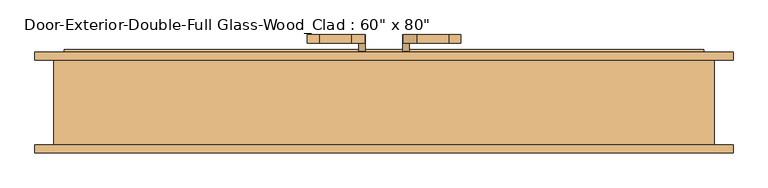
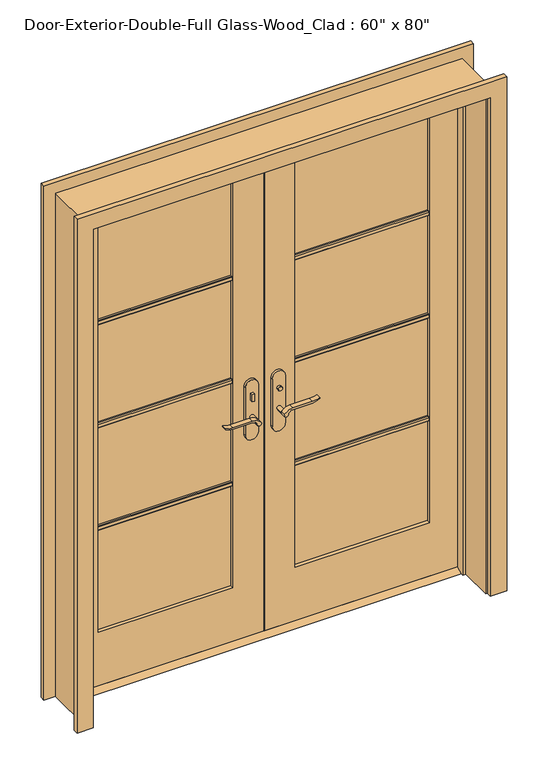
"""IFC4 building model written with IfcOpenShell, lengths in millimetres: door geometry."""

import ifcopenshell
import ifcopenshell.guid

model = None  # the IFC model being written
_history = None  # IfcOwnerHistory: only IFC2X3 demands one
_inside = {}  # id of a spatial element -> (the spatial element, [elements in it])
_under = {}  # id of a project, library or spatial element -> (it, [spatial elements below it])
_declared = {}  # id of a project -> (the project, [libraries it declares])
_typed = {}  # id of a type object -> (the type object, [elements of that type])
_made_of = {}  # id of a material, layer set ... -> (it, [elements and type objects made of it])


def new_model(schema):
    """Start an empty IFC model of exactly this schema.

    Asked for "IFC4X3", IfcOpenShell would pick the latest addendum, in which some entities
    have other attributes; the version numbers below select the first issue.
    IFC2X3 requires an IfcOwnerHistory on every rooted entity: one is made here for all.
    """
    global model, _history
    if schema == "IFC4X3":
        model = ifcopenshell.file(schema_version=(4, 3, 0, 0))
    else:
        model = ifcopenshell.file(schema=schema)
    _inside.clear()
    _under.clear()
    _declared.clear()
    _typed.clear()
    _made_of.clear()
    _history = None
    if model.schema == "IFC2X3":
        org = make("IfcOrganization", Name="unknown")
        user = make(
            "IfcPersonAndOrganization",
            ThePerson=make("IfcPerson", FamilyName="unknown"),
            TheOrganization=org,
        )
        app = make(
            "IfcApplication",
            ApplicationDeveloper=org,
            Version="unknown",
            ApplicationFullName="unknown",
            ApplicationIdentifier="unknown",
        )
        _history = make(
            "IfcOwnerHistory",
            OwningUser=user,
            OwningApplication=app,
            ChangeAction="ADDED",
            CreationDate=0,
        )
    return model


def make(cls, **values):
    """One entity of the class cls with the attributes given. An attribute that is None is left unset."""
    return model.create_entity(
        cls, **{name: value for name, value in values.items() if value is not None}
    )


def rooted(cls, **values):
    """An entity with a GlobalId (a new one), such as an element, a storey or a relation."""
    return make(cls, GlobalId=ifcopenshell.guid.new(), OwnerHistory=_history, **values)


def si_unit(unit_type, name, prefix=None):
    """IfcSIUnit, for example si_unit("LENGTHUNIT", "METRE", prefix="MILLI")."""
    return make("IfcSIUnit", UnitType=unit_type, Prefix=prefix, Name=name)


def assignment(units):
    """IfcUnitAssignment: the units of a project."""
    return None if units is None else make("IfcUnitAssignment", Units=units)


def point(xyz):
    """IfcCartesianPoint."""
    return None if xyz is None else make("IfcCartesianPoint", Coordinates=xyz)


def direction(xyz):
    """IfcDirection."""
    return None if xyz is None else make("IfcDirection", DirectionRatios=xyz)


def frame(location, z_axis=None, x_axis=None):
    """IfcAxis2Placement3D, a coordinate frame: its origin and axes. An axis left out is left unset."""
    return make(
        "IfcAxis2Placement3D",
        Location=point(location),
        Axis=direction(z_axis),
        RefDirection=direction(x_axis),
    )


def frame_2d(location, x_axis=None):
    """IfcAxis2Placement2D, a coordinate frame in the plane: its origin and x axis."""
    return make(
        "IfcAxis2Placement2D", Location=point(location), RefDirection=direction(x_axis)
    )


def origin():
    """The frame at (0, 0, 0) with its axes left unset."""
    return frame((0.0, 0.0, 0.0))


def place(relative_to, where):
    """IfcLocalPlacement: puts the frame where relative to a parent placement (None: the world)."""
    return make(
        "IfcLocalPlacement", PlacementRelTo=relative_to, RelativePlacement=where
    )


def context(
    kind, dimensions, precision=None, world=None, true_north=None, identifier=None
):
    """IfcGeometricRepresentationContext, for example the 3D "Model" context."""
    return make(
        "IfcGeometricRepresentationContext",
        ContextIdentifier=identifier,
        ContextType=kind,
        CoordinateSpaceDimension=dimensions,
        Precision=precision,
        WorldCoordinateSystem=world,
        TrueNorth=true_north,
    )


def project(units=None, contexts=None):
    """IfcProject with its units and contexts."""
    return rooted(
        "IfcProject",
        Name="project",
        RepresentationContexts=contexts,
        UnitsInContext=assignment(units),
    )


def spatial(cls, under=None, at=None, **own):
    """A site, building, storey or space (cls), placed at a placement, below another one or the project."""
    s = rooted(cls, ObjectPlacement=at, **own)
    if under is not None:
        _under.setdefault(under.id(), (under, []))[1].append(s)
    return s


def polyline(points):
    """IfcPolyline through the points."""
    return make("IfcPolyline", Points=[point(p) for p in points])


def circle_curve(where, radius):
    """IfcCircle in the frame where."""
    return make("IfcCircle", Position=where, Radius=radius)


def trimmed(basis, trim1, trim2, sense, master):
    """IfcTrimmedCurve: the piece of a basis curve between two trims."""
    return make(
        "IfcTrimmedCurve",
        BasisCurve=basis,
        Trim1=trim1,
        Trim2=trim2,
        SenseAgreement=sense,
        MasterRepresentation=master,
    )


def segment(curve, same_sense, transition):
    """IfcCompositeCurveSegment."""
    return make(
        "IfcCompositeCurveSegment",
        Transition=transition,
        SameSense=same_sense,
        ParentCurve=curve,
    )


def composite_curve(segments, self_intersect=None):
    """IfcCompositeCurve: segments joined end to end."""
    return make("IfcCompositeCurve", Segments=segments, SelfIntersect=self_intersect)


def outline(outer, holes=None, kind="AREA"):
    """IfcArbitraryClosedProfileDef: a profile drawn as a closed curve; with holes, ...WithVoids."""
    if holes is None:
        return make("IfcArbitraryClosedProfileDef", ProfileType=kind, OuterCurve=outer)
    return make(
        "IfcArbitraryProfileDefWithVoids",
        ProfileType=kind,
        OuterCurve=outer,
        InnerCurves=holes,
    )


def extrude(swept, where, along, depth):
    """IfcExtrudedAreaSolid: the profile swept, set in the frame where, extruded along a direction by depth."""
    return make(
        "IfcExtrudedAreaSolid",
        SweptArea=swept,
        Position=where,
        ExtrudedDirection=direction(along),
        Depth=depth,
    )


def faces_of(points, faces, orient=None, outer=None):
    """IfcFace entities. A face is a list of loops; a loop is a list of indices into points, from 0.

    orient and outer hold one flag for each loop. By default every Orientation is true, the
    first loop of a face is its IfcFaceOuterBound and the others are IfcFaceBound.
    """
    made = []
    for i, loops in enumerate(faces):
        bounds = []
        for j, loop in enumerate(loops):
            is_outer = j == 0 if outer is None else outer[i][j]
            bounds.append(
                make(
                    "IfcFaceOuterBound" if is_outer else "IfcFaceBound",
                    Bound=make("IfcPolyLoop", Polygon=[points[k] for k in loop]),
                    Orientation=True if orient is None else orient[i][j],
                )
            )
        made.append(make("IfcFace", Bounds=bounds))
    return made


def faceted_brep(points, faces, orient=None, outer=None, voids=None):
    """IfcFacetedBrep: a solid bounded by flat faces; with voids (closed shells), ...WithVoids."""
    shared = [point(p) for p in points]
    hull = make("IfcClosedShell", CfsFaces=faces_of(shared, faces, orient, outer))
    if voids is None:
        return make("IfcFacetedBrep", Outer=hull)
    return make(
        "IfcFacetedBrepWithVoids",
        Outer=hull,
        Voids=[
            make(cls, CfsFaces=faces_of(shared, fs, o, b)) for cls, fs, o, b in voids
        ],
    )


def shape(context_of_items, identifier, shape_type, items):
    """IfcShapeRepresentation: the items that make up one representation, for example the "Body"."""
    return make(
        "IfcShapeRepresentation",
        ContextOfItems=context_of_items,
        RepresentationIdentifier=identifier,
        RepresentationType=shape_type,
        Items=items,
    )


def source(mapping_origin, context_of_items, identifier, shape_type, items):
    """IfcRepresentationMap: a shape defined once, which mapped items show again and again."""
    return make(
        "IfcRepresentationMap",
        MappingOrigin=mapping_origin,
        MappedRepresentation=shape(context_of_items, identifier, shape_type, items),
    )


def transform(
    local_origin,
    x_axis=None,
    y_axis=None,
    z_axis=None,
    scale=None,
    scale2=None,
    scale3=None,
    uniform=True,
):
    """IfcCartesianTransformationOperator3D, or its non-uniform kind. x_axis, y_axis, z_axis: its Axis1, 2, 3."""
    if uniform:
        return make(
            "IfcCartesianTransformationOperator3D",
            Axis1=direction(x_axis),
            Axis2=direction(y_axis),
            LocalOrigin=point(local_origin),
            Scale=scale,
            Axis3=direction(z_axis),
        )
    return make(
        "IfcCartesianTransformationOperator3DnonUniform",
        Axis1=direction(x_axis),
        Axis2=direction(y_axis),
        LocalOrigin=point(local_origin),
        Scale=scale,
        Axis3=direction(z_axis),
        Scale2=scale2,
        Scale3=scale3,
    )


def mapped(mapping_source, mapping_target):
    """IfcMappedItem: shows the shape of a source again, moved by a transform."""
    return make(
        "IfcMappedItem", MappingSource=mapping_source, MappingTarget=mapping_target
    )


def made_of(thing, what):
    """Note that an element or type object is made of a material, layer set ...; save() writes the relation."""
    if what is not None:
        _made_of.setdefault(what.id(), (what, []))[1].append(thing)
    return thing


def element(
    cls,
    number,
    at=None,
    inside=None,
    cuts=None,
    type_object=None,
    material=None,
    context=None,
    identifier="Body",
    shape_type=None,
    held_by="IfcProductDefinitionShape",
    body=None,
    shapes=None,
    **own,
):
    """One element of the class cls, such as IfcWall. Its Tag is "e" and its number.

    at: its placement. inside: the storey or other place that contains it. cuts: it is an
    opening in that element (IfcRelVoidsElement). A single representation is given by context,
    identifier, shape_type and body (its items); several are given by shapes. held_by: the class
    of the entity that holds the representations. save() writes the other relations.
    """
    e = rooted(cls, Tag="e%d" % number, ObjectPlacement=at, **own)
    if body is not None:
        shapes = [shape(context, identifier, shape_type, body)]
    if shapes is not None:
        e.Representation = make(held_by, Representations=shapes)
    if inside is not None:
        _inside.setdefault(inside.id(), (inside, []))[1].append(e)
    if cuts is not None:
        rooted(
            "IfcRelVoidsElement", RelatingBuildingElement=cuts, RelatedOpeningElement=e
        )
    if type_object is not None:
        _typed.setdefault(type_object.id(), (type_object, []))[1].append(e)
    return made_of(e, material)


def aggregate(whole, parts):
    """IfcRelAggregates: a whole, such as a stair, and the parts it consists of."""
    return rooted("IfcRelAggregates", RelatingObject=whole, RelatedObjects=parts)


def save(model, path):
    """Write the relations noted so far, then the file.

    IfcRelAggregates (storeys below a building ...), IfcRelContainedInSpatialStructure (elements
    in a storey), IfcRelDefinesByType, IfcRelAssociatesMaterial and IfcRelDeclares: one each for
    every whole, place, type object, material and project.
    """
    for whole, parts in _under.values():
        aggregate(whole, parts)
    for where, things in _inside.values():
        rooted(
            "IfcRelContainedInSpatialStructure",
            RelatedElements=things,
            RelatingStructure=where,
        )
    for kind, things in _typed.values():
        rooted("IfcRelDefinesByType", RelatedObjects=things, RelatingType=kind)
    for what, things in _made_of.values():
        rooted("IfcRelAssociatesMaterial", RelatedObjects=things, RelatingMaterial=what)
    for by, libraries in _declared.values():
        rooted("IfcRelDeclares", RelatingContext=by, RelatedDefinitions=libraries)
    model.write(path)


def door_b03bd389(model_context):
    return source(origin(), model_context, "Body", "SolidModel", [
        extrude(outline(polyline([(63.5, 12.7), (98.425, 12.7), (123.825, 0.0), (38.1, 0.0), (63.5, 12.7)])), frame((-762.0, 0.0, 0.0), z_axis=(1.0, 0.0, 0.0), x_axis=(0.0, 1.0, 0.0)), (0.0, 0.0, 1.0), 1524.0),
        extrude(outline(polyline([(-47.4019111, 43.5), (-57.4019111, 43.5), (-57.4019111, 53.5), (-47.4019111, 53.5), (-47.4019111, 43.5)])), frame((0.0, 0.0, 981.9), z_axis=(0.0, 0.0, 1.0), x_axis=(1.0, 0.0, 0.0)), (0.0, 0.0, 1.0), 30.0),
        extrude(outline(composite_curve([segment(trimmed(circle_curve(frame_2d((996.9, -52.4019111)), 8.0), [point((996.9, -60.4019111))], [point((996.9, -44.4019111))], False, "CARTESIAN"), True, "CONTINUOUS"), segment(trimmed(circle_curve(frame_2d((996.9, -52.4019111)), 8.0), [point((996.9, -44.4019111))], [point((996.9, -60.4019111))], False, "CARTESIAN"), True, "CONTINUOUS")], self_intersect=False)), frame((0.0, 108.425, 0.0), z_axis=(0.0, 1.0, 0.0), x_axis=(0.0, 0.0, 1.0)), (0.0, 0.0, 1.0), 10.0),
        extrude(outline(composite_curve([segment(trimmed(circle_curve(frame_2d((897.1555521, -76.0694241)), 37.2832219), [point((919.0523287, -45.8937749))], [point((934.4, -77.7693445))], False, "CARTESIAN"), True, "CONTINUOUS"), segment(polyline([(934.4, -77.7693445), (934.4, -154.045502)]), True, "CONTINUOUS"), segment(trimmed(circle_curve(frame_2d((1017.6850638, -153.9791202)), 83.2850902), [point((934.4, -154.045502))], [point((939.4, -182.4019111))], True, "CARTESIAN"), True, "CONTINUOUS"), segment(polyline([(939.4, -182.4019111), (936.6135558, -182.4019111)]), True, "CONTINUOUS"), segment(trimmed(circle_curve(frame_2d((986.6709207, -150.4622499)), 59.3791355), [point((936.6135558, -182.4019111))], [point((927.4, -154.045502))], False, "CARTESIAN"), True, "CONTINUOUS"), segment(polyline([(927.4, -154.045502), (927.4, -77.7881013)]), True, "CONTINUOUS"), segment(trimmed(circle_curve(frame_2d((909.2738613, -77.7881013)), 18.1261387), [point((927.4, -77.7881013))], [point((914.4, -60.4019111))], True, "CARTESIAN"), True, "CONTINUOUS"), segment(trimmed(circle_curve(frame_2d((914.4, -52.4019111)), 8.0), [point((914.4, -60.4019111))], [point((919.0523287, -45.8937749))], False, "CARTESIAN"), True, "CONTINUOUS")], self_intersect=False)), frame((0.0, 3.5, 0.0), z_axis=(0.0, 1.0, 0.0), x_axis=(0.0, 0.0, 1.0)), (0.0, 0.0, 1.0), 20.0),
        extrude(outline(composite_curve([segment(trimmed(circle_curve(frame_2d((914.4, -52.4019111)), 8.0), [point((914.3999903, -60.4019111))], [point((919.0523287, -45.8937749))], False, "CARTESIAN"), True, "CONTINUOUS"), segment(trimmed(circle_curve(frame_2d((897.1555521, -76.0694241)), 37.2832219), [point((919.0523287, -45.8937749))], [point((934.4, -77.7693445))], False, "CARTESIAN"), True, "CONTINUOUS"), segment(polyline([(934.4, -77.7693445), (934.4, -154.045502)]), True, "CONTINUOUS"), segment(trimmed(circle_curve(frame_2d((1017.6850638, -153.9791202)), 83.2850902), [point((934.4, -154.045502))], [point((939.4, -182.4019111))], True, "CARTESIAN"), True, "CONTINUOUS"), segment(polyline([(939.4, -182.4019111), (936.6135558, -182.4019111)]), True, "CONTINUOUS"), segment(trimmed(circle_curve(frame_2d((986.6709207, -150.4622499)), 59.3791355), [point((936.6135558, -182.4019111))], [point((927.4, -154.045502))], False, "CARTESIAN"), True, "CONTINUOUS"), segment(polyline([(927.4, -154.045502), (927.4, -77.788099)]), True, "CONTINUOUS"), segment(trimmed(circle_curve(frame_2d((909.2738682, -77.788099)), 18.1261318), [point((927.4, -77.788099))], [point((914.3999903, -60.4019111))], True, "CARTESIAN"), True, "CONTINUOUS")], self_intersect=False)), frame((0.0, 138.425, 0.0), z_axis=(0.0, 1.0, 0.0), x_axis=(0.0, 0.0, 1.0)), (0.0, 0.0, 1.0), 20.0),
        extrude(outline(composite_curve([segment(trimmed(circle_curve(frame_2d((914.4, -52.4019111)), 8.0), [point((914.4, -60.4019111))], [point((914.4, -44.4019111))], False, "CARTESIAN"), True, "CONTINUOUS"), segment(trimmed(circle_curve(frame_2d((914.4, -52.4019111)), 8.0), [point((914.4, -44.4019111))], [point((914.4, -60.4019111))], False, "CARTESIAN"), True, "CONTINUOUS")], self_intersect=False)), frame((0.0, 23.5, 0.0), z_axis=(0.0, 1.0, 0.0), x_axis=(0.0, 0.0, 1.0)), (0.0, 0.0, 1.0), 30.0),
        extrude(outline(composite_curve([segment(trimmed(circle_curve(frame_2d((914.4, -52.4019111)), 8.0), [point((914.4, -60.4019111))], [point((914.4, -44.4019111))], False, "CARTESIAN"), True, "CONTINUOUS"), segment(trimmed(circle_curve(frame_2d((914.4, -52.4019111)), 8.0), [point((914.4, -44.4019111))], [point((914.4, -60.4019111))], False, "CARTESIAN"), True, "CONTINUOUS")], self_intersect=False)), frame((0.0, 108.425, 0.0), z_axis=(0.0, 1.0, 0.0), x_axis=(0.0, 0.0, 1.0)), (0.0, 0.0, 1.0), 30.0),
        extrude(outline(composite_curve([segment(polyline([(844.4, -27.4019111), (1039.4, -27.4019111)]), True, "CONTINUOUS"), segment(trimmed(circle_curve(frame_2d((1039.4, -52.4019111)), 25.0), [point((1039.4, -27.4019111))], [point((1039.4, -77.4019111))], False, "CARTESIAN"), True, "CONTINUOUS"), segment(polyline([(1039.4, -77.4019111), (844.4, -77.4019111)]), True, "CONTINUOUS"), segment(trimmed(circle_curve(frame_2d((844.4, -52.4019111)), 25.0), [point((844.4, -77.4019111))], [point((844.4, -27.4019111))], False, "CARTESIAN"), True, "CONTINUOUS")], self_intersect=False)), frame((0.0, 53.5, 0.0), z_axis=(0.0, 1.0, 0.0), x_axis=(0.0, 0.0, 1.0)), (0.0, 0.0, 1.0), 10.0),
        extrude(outline(composite_curve([segment(polyline([(844.4, -27.4019111), (1039.4, -27.4019111)]), True, "CONTINUOUS"), segment(trimmed(circle_curve(frame_2d((1039.4, -52.4019111)), 25.0), [point((1039.4, -27.4019111))], [point((1039.4, -77.4019111))], False, "CARTESIAN"), True, "CONTINUOUS"), segment(polyline([(1039.4, -77.4019111), (844.4, -77.4019111)]), True, "CONTINUOUS"), segment(trimmed(circle_curve(frame_2d((844.4, -52.4019111)), 25.0), [point((844.4, -77.4019111))], [point((844.4, -27.4019111))], False, "CARTESIAN"), True, "CONTINUOUS")], self_intersect=False)), frame((0.0, 98.425, 0.0), z_axis=(0.0, 1.0, 0.0), x_axis=(0.0, 0.0, 1.0)), (0.0, 0.0, 1.0), 10.0),
        extrude(outline(polyline([(47.3875, 118.425), (57.3875, 118.425), (57.3875, 108.425), (47.3875, 108.425), (47.3875, 118.425)])), frame((0.0, 0.0, 981.9), z_axis=(0.0, 0.0, 1.0), x_axis=(1.0, 0.0, 0.0)), (0.0, 0.0, 1.0), 30.0),
        extrude(outline(composite_curve([segment(trimmed(circle_curve(frame_2d((996.9, 52.3875)), 8.0), [point((996.9, 60.3875))], [point((996.9, 44.3875))], False, "CARTESIAN"), True, "CONTINUOUS"), segment(trimmed(circle_curve(frame_2d((996.9, 52.3875)), 8.0), [point((996.9, 44.3875))], [point((996.9, 60.3875))], False, "CARTESIAN"), True, "CONTINUOUS")], self_intersect=False)), frame((0.0, 43.5, 0.0), z_axis=(0.0, 1.0, 0.0), x_axis=(0.0, 0.0, 1.0)), (0.0, 0.0, 1.0), 10.0),
        extrude(outline(composite_curve([segment(trimmed(circle_curve(frame_2d((914.4, 52.3875)), 8.0), [point((919.0523287, 45.8793637))], [point((914.4, 60.3875))], False, "CARTESIAN"), True, "CONTINUOUS"), segment(trimmed(circle_curve(frame_2d((909.2738613, 77.7736901)), 18.1261387), [point((914.4, 60.3875))], [point((927.4, 77.7736901))], True, "CARTESIAN"), True, "CONTINUOUS"), segment(polyline([(927.4, 77.7736901), (927.4, 154.0310909)]), True, "CONTINUOUS"), segment(trimmed(circle_curve(frame_2d((986.6709207, 150.4478388)), 59.3791355), [point((927.4, 154.0310909))], [point((936.6135558, 182.3875))], False, "CARTESIAN"), True, "CONTINUOUS"), segment(polyline([(936.6135558, 182.3875), (939.4, 182.3875)]), True, "CONTINUOUS"), segment(trimmed(circle_curve(frame_2d((1017.6850638, 153.9647091)), 83.2850902), [point((939.4, 182.3875))], [point((934.4, 154.0310909))], True, "CARTESIAN"), True, "CONTINUOUS"), segment(polyline([(934.4, 154.0310909), (934.4, 77.7549333)]), True, "CONTINUOUS"), segment(trimmed(circle_curve(frame_2d((897.1555521, 76.0550129)), 37.2832219), [point((934.4, 77.7549333))], [point((919.0523287, 45.8793637))], False, "CARTESIAN"), True, "CONTINUOUS")], self_intersect=False)), frame((0.0, 138.425, 0.0), z_axis=(0.0, 1.0, 0.0), x_axis=(0.0, 0.0, 1.0)), (0.0, 0.0, 1.0), 20.0),
        extrude(outline(composite_curve([segment(trimmed(circle_curve(frame_2d((909.2738682, 77.7736878)), 18.1261318), [point((914.3999903, 60.3875))], [point((927.4, 77.7736878))], True, "CARTESIAN"), True, "CONTINUOUS"), segment(polyline([(927.4, 77.7736878), (927.4, 154.0310909)]), True, "CONTINUOUS"), segment(trimmed(circle_curve(frame_2d((986.6709207, 150.4478388)), 59.3791355), [point((927.4, 154.0310909))], [point((936.6135558, 182.3875))], False, "CARTESIAN"), True, "CONTINUOUS"), segment(polyline([(936.6135558, 182.3875), (939.4, 182.3875)]), True, "CONTINUOUS"), segment(trimmed(circle_curve(frame_2d((1017.6850638, 153.9647091)), 83.2850902), [point((939.4, 182.3875))], [point((934.4, 154.0310909))], True, "CARTESIAN"), True, "CONTINUOUS"), segment(polyline([(934.4, 154.0310909), (934.4, 77.7549333)]), True, "CONTINUOUS"), segment(trimmed(circle_curve(frame_2d((897.1555521, 76.0550129)), 37.2832219), [point((934.4, 77.7549333))], [point((919.0523287, 45.8793637))], False, "CARTESIAN"), True, "CONTINUOUS"), segment(trimmed(circle_curve(frame_2d((914.4, 52.3875)), 8.0), [point((919.0523287, 45.8793637))], [point((914.3999903, 60.3875))], False, "CARTESIAN"), True, "CONTINUOUS")], self_intersect=False)), frame((0.0, 3.5, 0.0), z_axis=(0.0, 1.0, 0.0), x_axis=(0.0, 0.0, 1.0)), (0.0, 0.0, 1.0), 20.0),
        extrude(outline(composite_curve([segment(trimmed(circle_curve(frame_2d((914.4, 52.3875)), 8.0), [point((914.4, 60.3875))], [point((914.4, 44.3875))], False, "CARTESIAN"), True, "CONTINUOUS"), segment(trimmed(circle_curve(frame_2d((914.4, 52.3875)), 8.0), [point((914.4, 44.3875))], [point((914.4, 60.3875))], False, "CARTESIAN"), True, "CONTINUOUS")], self_intersect=False)), frame((0.0, 108.425, 0.0), z_axis=(0.0, 1.0, 0.0), x_axis=(0.0, 0.0, 1.0)), (0.0, 0.0, 1.0), 30.0),
        extrude(outline(composite_curve([segment(trimmed(circle_curve(frame_2d((914.4, 52.3875)), 8.0), [point((914.4, 60.3875))], [point((914.4, 44.3875))], False, "CARTESIAN"), True, "CONTINUOUS"), segment(trimmed(circle_curve(frame_2d((914.4, 52.3875)), 8.0), [point((914.4, 44.3875))], [point((914.4, 60.3875))], False, "CARTESIAN"), True, "CONTINUOUS")], self_intersect=False)), frame((0.0, 23.5, 0.0), z_axis=(0.0, 1.0, 0.0), x_axis=(0.0, 0.0, 1.0)), (0.0, 0.0, 1.0), 30.0),
        extrude(outline(composite_curve([segment(trimmed(circle_curve(frame_2d((844.4, 52.3875)), 25.0), [point((844.4, 27.3875))], [point((844.4, 77.3875))], False, "CARTESIAN"), True, "CONTINUOUS"), segment(polyline([(844.4, 77.3875), (1039.4, 77.3875)]), True, "CONTINUOUS"), segment(trimmed(circle_curve(frame_2d((1039.4, 52.3875)), 25.0), [point((1039.4, 77.3875))], [point((1039.4, 27.3875))], False, "CARTESIAN"), True, "CONTINUOUS"), segment(polyline([(1039.4, 27.3875), (844.4, 27.3875)]), True, "CONTINUOUS")], self_intersect=False)), frame((0.0, 98.425, 0.0), z_axis=(0.0, 1.0, 0.0), x_axis=(0.0, 0.0, 1.0)), (0.0, 0.0, 1.0), 10.0),
        extrude(outline(composite_curve([segment(trimmed(circle_curve(frame_2d((844.4, 52.3875)), 25.0), [point((844.4, 27.3875))], [point((844.4, 77.3875))], False, "CARTESIAN"), True, "CONTINUOUS"), segment(polyline([(844.4, 77.3875), (1039.4, 77.3875)]), True, "CONTINUOUS"), segment(trimmed(circle_curve(frame_2d((1039.4, 52.3875)), 25.0), [point((1039.4, 77.3875))], [point((1039.4, 27.3875))], False, "CARTESIAN"), True, "CONTINUOUS"), segment(polyline([(1039.4, 27.3875), (844.4, 27.3875)]), True, "CONTINUOUS")], self_intersect=False)), frame((0.0, 53.5, 0.0), z_axis=(0.0, 1.0, 0.0), x_axis=(0.0, 0.0, 1.0)), (0.0, 0.0, 1.0), 10.0),
        extrude(outline(polyline([(77.47, 1502.171875), (77.47, 1483.121875), (71.12, 1483.121875), (67.945, 1486.296875), (67.945, 1498.996875), (71.12, 1502.171875), (77.47, 1502.171875)])), frame((120.65, 0.0, 0.0), z_axis=(1.0, 0.0, 0.0), x_axis=(0.0, 1.0, 0.0)), (0.0, 0.0, 1.0), 520.7),
        extrude(outline(polyline([(77.47, 1081.88125), (77.47, 1062.83125), (71.12, 1062.83125), (67.945, 1066.00625), (67.945, 1078.70625), (71.12, 1081.88125), (77.47, 1081.88125)])), frame((120.65, 0.0, 0.0), z_axis=(1.0, 0.0, 0.0), x_axis=(0.0, 1.0, 0.0)), (0.0, 0.0, 1.0), 520.7),
        extrude(outline(polyline([(77.47, 661.590625), (77.47, 642.540625), (71.12, 642.540625), (67.945, 645.715625), (67.945, 658.415625), (71.12, 661.590625), (77.47, 661.590625)])), frame((120.65, 0.0, 0.0), z_axis=(1.0, 0.0, 0.0), x_axis=(0.0, 1.0, 0.0)), (0.0, 0.0, 1.0), 520.7),
        extrude(outline(polyline([(84.455, 1502.171875), (90.805, 1502.171875), (93.98, 1498.996875), (93.98, 1486.296875), (90.805, 1483.121875), (84.455, 1483.121875), (84.455, 1502.171875)])), frame((-641.35, 0.0, 0.0), z_axis=(1.0, 0.0, 0.0), x_axis=(0.0, 1.0, 0.0)), (0.0, 0.0, 1.0), 520.7),
        extrude(outline(polyline([(84.455, 1081.88125), (90.805, 1081.88125), (93.98, 1078.70625), (93.98, 1066.00625), (90.805, 1062.83125), (84.455, 1062.83125), (84.455, 1081.88125)])), frame((-641.35, 0.0, 0.0), z_axis=(1.0, 0.0, 0.0), x_axis=(0.0, 1.0, 0.0)), (0.0, 0.0, 1.0), 520.7),
        extrude(outline(polyline([(84.455, 661.590625), (90.805, 661.590625), (93.98, 658.415625), (93.98, 645.715625), (90.805, 642.540625), (84.455, 642.540625), (84.455, 661.590625)])), frame((-641.35, 0.0, 0.0), z_axis=(1.0, 0.0, 0.0), x_axis=(0.0, 1.0, 0.0)), (0.0, 0.0, 1.0), 520.7),
        extrude(outline(polyline([(84.455, 1502.171875), (90.805, 1502.171875), (93.98, 1498.996875), (93.98, 1486.296875), (90.805, 1483.121875), (84.455, 1483.121875), (84.455, 1502.171875)])), frame((120.65, 0.0, 0.0), z_axis=(1.0, 0.0, 0.0), x_axis=(0.0, 1.0, 0.0)), (0.0, 0.0, 1.0), 520.7),
        extrude(outline(polyline([(84.455, 1081.88125), (90.805, 1081.88125), (93.98, 1078.70625), (93.98, 1066.00625), (90.805, 1062.83125), (84.455, 1062.83125), (84.455, 1081.88125)])), frame((120.65, 0.0, 0.0), z_axis=(1.0, 0.0, 0.0), x_axis=(0.0, 1.0, 0.0)), (0.0, 0.0, 1.0), 520.7),
        extrude(outline(polyline([(84.455, 661.590625), (90.805, 661.590625), (93.98, 658.415625), (93.98, 645.715625), (90.805, 642.540625), (84.455, 642.540625), (84.455, 661.590625)])), frame((120.65, 0.0, 0.0), z_axis=(1.0, 0.0, 0.0), x_axis=(0.0, 1.0, 0.0)), (0.0, 0.0, 1.0), 520.7),
        extrude(outline(polyline([(77.47, 1502.171875), (77.47, 1483.121875), (71.12, 1483.121875), (67.945, 1486.296875), (67.945, 1498.996875), (71.12, 1502.171875), (77.47, 1502.171875)])), frame((-641.35, 0.0, 0.0), z_axis=(1.0, 0.0, 0.0), x_axis=(0.0, 1.0, 0.0)), (0.0, 0.0, 1.0), 520.7),
        extrude(outline(polyline([(77.47, 1081.88125), (77.47, 1062.83125), (71.12, 1062.83125), (67.945, 1066.00625), (67.945, 1078.70625), (71.12, 1081.88125), (77.47, 1081.88125)])), frame((-641.35, 0.0, 0.0), z_axis=(1.0, 0.0, 0.0), x_axis=(0.0, 1.0, 0.0)), (0.0, 0.0, 1.0), 520.7),
        extrude(outline(polyline([(77.47, 661.590625), (77.47, 642.540625), (71.12, 642.540625), (67.945, 645.715625), (67.945, 658.415625), (71.12, 661.590625), (77.47, 661.590625)])), frame((-641.35, 0.0, 0.0), z_axis=(1.0, 0.0, 0.0), x_axis=(0.0, 1.0, 0.0)), (0.0, 0.0, 1.0), 520.7),
        extrude(outline(polyline([(0.0, 768.35), (0.0, 831.85), (2101.85, 831.85), (2101.85, -831.85), (0.0, -831.85), (0.0, -768.35), (2038.35, -768.35), (2038.35, 768.35), (0.0, 768.35)])), frame((0.0, 98.425, 0.0), z_axis=(0.0, 1.0, 0.0), x_axis=(0.0, 0.0, 1.0)), (0.0, 0.0, 1.0), 19.05),
        extrude(outline(polyline([(0.0, 768.35), (0.0, 831.85), (2101.85, 831.85), (2101.85, -831.85), (0.0, -831.85), (0.0, -768.35), (2038.35, -768.35), (2038.35, 768.35), (0.0, 768.35)])), frame((0.0, -123.825, 0.0), z_axis=(0.0, 1.0, 0.0), x_axis=(0.0, 0.0, 1.0)), (0.0, 0.0, 1.0), 19.05),
        extrude(outline(polyline([(12.7, 762.0), (2032.0, 762.0), (2032.0, 1.5875), (12.7, 1.5875), (12.7, 762.0)]), holes=[polyline([(1912.9375, 120.65), (1912.9375, 641.35), (231.775, 641.35), (231.775, 120.65), (1912.9375, 120.65)])]), frame((0.0, 63.5, 0.0), z_axis=(0.0, 1.0, 0.0), x_axis=(0.0, 0.0, 1.0)), (0.0, 0.0, 1.0), 34.925),
        extrude(outline(polyline([(2032.0, -762.0), (12.7, -762.0), (12.7, -1.6019111), (2032.0, -1.6019111), (2032.0, -762.0)]), holes=[polyline([(231.775, -641.35), (1912.9375, -641.35), (1912.9375, -120.65), (231.775, -120.65), (231.775, -641.35)])]), frame((0.0, 63.5, 0.0), z_axis=(0.0, 1.0, 0.0), x_axis=(0.0, 0.0, 1.0)), (0.0, 0.0, 1.0), 34.925),
        faceted_brep([(787.4, 98.425, 0.0), (787.4, -104.775, 0.0), (762.0, -104.775, 0.0), (762.0, 28.575, 0.0), (749.3, 28.575, 0.0), (749.3, 63.5, 0.0), (762.0, 63.5, 0.0), (762.0, 98.425, 0.0), (787.4, 98.425, 2057.4), (787.4, -104.775, 2057.4), (-787.4, -104.775, 2057.4), (-787.4, -104.775, 0.0), (-762.0, -104.775, 0.0), (-762.0, -104.775, 2032.0), (762.0, -104.775, 2032.0), (762.0, 28.575, 2032.0), (-762.0, 28.575, 2032.0), (-762.0, 28.575, 0.0), (-749.3, 28.575, 0.0), (-749.3, 28.575, 2019.3), (749.3, 28.575, 2019.3), (749.3, 63.5, 2019.3), (1.5875, 63.5, 2019.3), (-1.6019111, 63.5, 2019.3), (-749.3, 63.5, 2019.3), (-749.3, 63.5, 0.0), (-762.0, 63.5, 0.0), (-762.0, 63.5, 2032.0), (-1.6019111, 63.5, 2032.0), (1.5875, 63.5, 2032.0), (762.0, 63.5, 2032.0), (762.0, 98.425, 2032.0), (1.5875, 98.425, 2032.0), (-1.6019111, 98.425, 2032.0), (-762.0, 98.425, 2032.0), (-762.0, 98.425, 0.0), (-787.4, 98.425, 0.0), (-787.4, 98.425, 2057.4)], [[[0, 1, 2, 3, 4, 5, 6, 7]], [[1, 0, 8, 9]], [[2, 1, 9, 10, 11, 12, 13, 14]], [[3, 2, 14, 15]], [[4, 3, 15, 16, 17, 18, 19, 20]], [[5, 4, 20, 21]], [[6, 5, 21, 22, 23, 24, 25, 26, 27, 28, 29, 30]], [[7, 6, 30, 31]], [[0, 7, 31, 32, 33, 34, 35, 36, 37, 8]], [[9, 8, 37, 10]], [[14, 13, 16, 15]], [[20, 19, 24, 23, 22, 21]], [[31, 30, 29, 28, 27, 34, 33, 32]], [[12, 11, 36, 35, 26, 25, 18, 17]], [[11, 10, 37, 36]], [[13, 12, 17, 16]], [[19, 18, 25, 24]], [[27, 26, 35, 34]]]),
        extrude(outline(polyline([(641.35, 77.47), (120.65, 77.47), (120.65, 84.455), (641.35, 84.455), (641.35, 77.47)])), frame((0.0, 0.0, 231.775), z_axis=(0.0, 0.0, 1.0), x_axis=(1.0, 0.0, 0.0)), (0.0, 0.0, 1.0), 1681.1625),
        extrude(outline(polyline([(-120.65, 77.47), (-641.35, 77.47), (-641.35, 84.455), (-120.65, 84.455), (-120.65, 77.47)])), frame((0.0, 0.0, 231.775), z_axis=(0.0, 0.0, 1.0), x_axis=(1.0, 0.0, 0.0)), (0.0, 0.0, 1.0), 1681.1625),
    ])


if __name__ == "__main__":
    model = new_model("IFC4")
    model_context = context("Model", 3, world=origin())
    ifc_project = project(units=[si_unit("LENGTHUNIT", "METRE", prefix="MILLI")], contexts=[model_context])
    site = spatial("IfcSite", under=ifc_project)
    building = spatial("IfcBuilding", under=site)
    placement = place(None, origin())
    door_shape = door_b03bd389(model_context)
    element("IfcDoor", 1, ObjectType="Door-Exterior-Double-Full Glass-Wood_Clad : 60\" x 80\"", at=placement, inside=building, context=model_context, shape_type="MappedRepresentation", body=[
        mapped(door_shape, transform((0.0, 0.0, 0.0), x_axis=(1.0, 0.0, 0.0), y_axis=(0.0, 1.0, 0.0), z_axis=(0.0, 0.0, 1.0))),
    ])
    save(model, "model.ifc")

# Revit data of these elements
# Project information
#   Project Issue Date = "Issue Date"
#   Project Status = "Project Status"
#   Client Name = "Owner"
#   Project Address = "Enter address here"
#   Project Name = "Project Name"
#   Project Number = "Project Number"
# Type "Door-Exterior-Double-Full Glass-Wood_Clad : 60\" x 80\""
#   Type Mark = "8"
#   Assembly Code = "B2030100"
#   Analytic Construction = "French door, wood frame with double glass"
#   Top Rail = 0' - 4 11/16"
#   Threshold Offset [instance default] = 0' - 0 1/2"
#   Thickness = 0' - 1 3/8"
#   Thermal Resistance (R) = 0.337392 (m²·K)/W
#   Swing Angle [instance default] = 90.00°
#   Stiles = 0' - 4 3/4"
#   Rough Width = 5' - 2"
#   Rough Height = 6' - 9"
#   Panel Width = 2' - 6"
#   Door Offset [instance default] = 0' - 0"
#   Height = 6' - 8"
#   Width = 5' - 0"
#   Heat Transfer Coefficient (U) = 2.96405 W/(m²·K)
#   Bottom Rail = 0' - 9 1/8"
#   Exterior Trim [instance default] = yes
#   Threshold [instance default] = yes
#   Show Grill [instance default] = yes
#   Function = 1
#   Trim Material = Cherry
#   Threshold Material = Cherry
#   Panel Material = Cherry
#   Glazing = Glass
#   Frame Material = Cherry
#   Door Handle Material = Aluminum
#   Visual Light Transmittance = 0
#   Solar Heat Gain Coefficient = 0
#   Wall Closure = (empty or 0)
#   Construction Type = (empty or 0)
# Element 1 (IfcDoor, "Door-Exterior-Double-Full Glass-Wood_Clad : 60\" x 80\"")
#   Materials on its faces: "Cherry", "Aluminum", "Glass"
# Materials
#   "Cherry": class "Wood", colour RGB 226 177 128, transparency 0, Description = "Prunus Serotina", Cost = 0
#   "Glass": class "Glass", colour RGB 0 128 192, transparency 0.75, Description = "Soda Lime Glass", Cost = 0
#   "Aluminum": class "Metal", colour RGB 247 247 247, transparency 0, Description = "Aluminum 6061", Cost = 0
